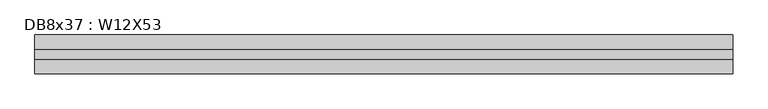
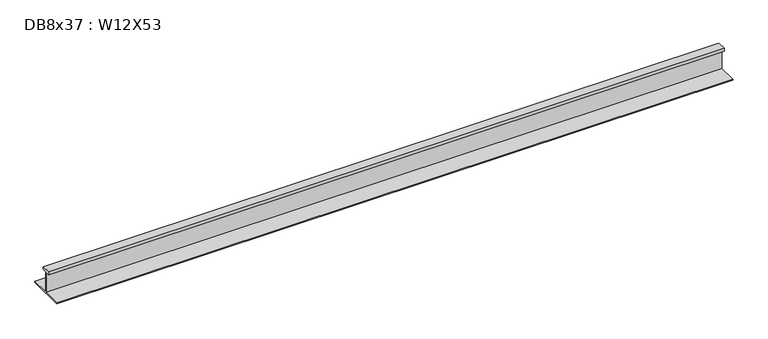
"""IFC4 building model written with IfcOpenShell, lengths in millimetres: beam geometry, DB8x37 : W12X53."""

from ifc_helpers import new_model, si_unit, frame, origin, place, context, project, spatial, polyline, outline, extrude, source, transform, mapped, element, save


def db8x37_w12x53_d4d5b842(model_context):
    return source(origin(), model_context, "Body", "SweptSolid", [
        extrude(outline(polyline([(38.1, 145.415), (38.1, 120.015), (2.921, 120.015), (2.921, -48.4505), (152.4, -48.4505), (152.4, -58.1025), (-152.4, -58.1025), (-152.4, -48.4505), (-2.921, -48.4505), (-2.921, 120.015), (-38.1, 120.015), (-38.1, 145.415), (38.1, 145.415)])), frame((-2731.008, 0.0, 0.0), z_axis=(1.0, 0.0, 0.0), x_axis=(0.0, 1.0, 0.0)), (0.0, 0.0, 1.0), 5462.016),
    ])


if __name__ == "__main__":
    model = new_model("IFC4")
    model_context = context("Model", 3, world=origin())
    ifc_project = project(units=[si_unit("LENGTHUNIT", "METRE", prefix="MILLI")], contexts=[model_context])
    site = spatial("IfcSite", under=ifc_project)
    building = spatial("IfcBuilding", under=site)
    placement = place(None, origin())
    db8x37_w12x53_shape = db8x37_w12x53_d4d5b842(model_context)
    element("IfcBeam", 1, ObjectType="DB8x37 : W12X53", at=placement, inside=building, context=model_context, shape_type="MappedRepresentation", body=[
        mapped(db8x37_w12x53_shape, transform((0.0, 0.0, 0.0), x_axis=(1.0, 0.0, 0.0), y_axis=(0.0, 1.0, 0.0), z_axis=(0.0, 0.0, 1.0))),
    ])
    save(model, "model.ifc")

# Revit data of these elements
# Type "DB8x37 : W12X53"
#   Assembly Code = "B10"
#   W = 53
#   Length [instance default] = 5' - 0"
#   bf = 0' - 10"
#   d = 1' - 0.1"
#   k = 0' - 1 3/8"
#   k2 = 0' - 0.8"
#   tf = 0' - 0.575"
#   tw = 0' - 0.345"
#   A = 0.108333 SF
#   Structural Material [instance default] = Steel ASTM A992
# Element 1 (IfcBeam, "DB8x37 : W12X53")
#   Materials on its faces: "Steel ASTM A992"
# Materials
#   "Steel ASTM A992": class "Metal", colour RGB 199 199 199, transparency 0, Description = "Structural steel 50ksi", Cost = 0
